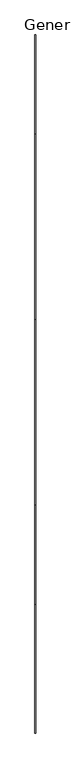
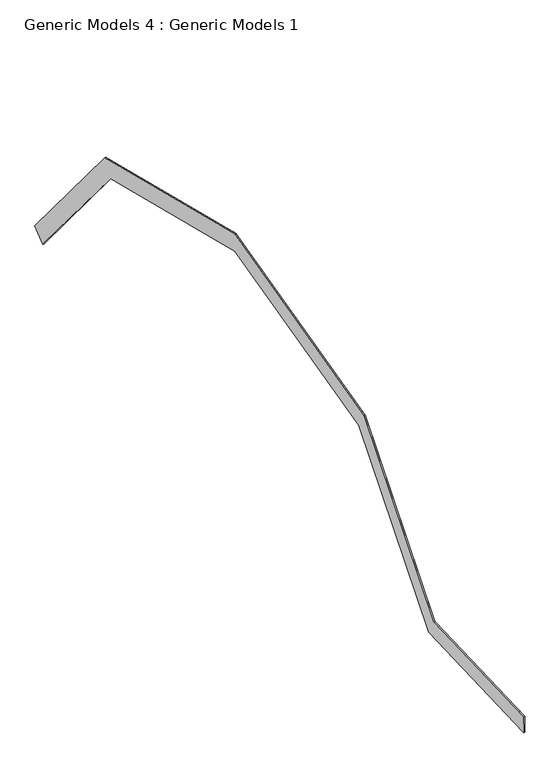
"""IFC4 building model written with IfcOpenShell, lengths in millimetres: proxy geometry, Generic Models 4 : Generic Models 1."""

from ifc_helpers import new_model, si_unit, frame, origin, place, context, project, spatial, polyline, outline, extrude, source, transform, mapped, element, save


def generic_models_4_generic_models_1_9f6939e7(model_context):
    return source(origin(), model_context, "Body", "SweptSolid", [
        extrude(outline(polyline([(11609.9309883, 2984.3405795), (10023.6412719, 4887.8882391), (7113.0570149, 5615.5343034), (4202.4384941, 4887.8796732), (2560.7151338, 2917.8116409), (331.5982071, 2831.1879261), (322.4759913, 3065.9329463), (2434.8673967, 3148.0206952), (4066.3626163, 5105.8149588), (7113.772024, 5867.6673107), (10161.1814316, 5105.8149588), (11797.360301, 3142.4003155), (11609.9309883, 2984.3405795)])), frame((29947.3870052, 0.0, 0.0), z_axis=(1.0, 0.0, 0.0), x_axis=(0.0, 1.0, 0.0)), (0.0, 0.0, 1.0), 13.5023771),
    ])


if __name__ == "__main__":
    model = new_model("IFC4")
    model_context = context("Model", 3, world=origin())
    ifc_project = project(units=[si_unit("LENGTHUNIT", "METRE", prefix="MILLI")], contexts=[model_context])
    site = spatial("IfcSite", under=ifc_project)
    building = spatial("IfcBuilding", under=site)
    placement = place(None, origin())
    generic_models_4_generic_models_1_shape = generic_models_4_generic_models_1_9f6939e7(model_context)
    element("IfcBuildingElementProxy", 1, Name="Generic Models 4 : Generic Models 1", ObjectType="Generic Models 4 : Generic Models 1", at=placement, inside=building, context=model_context, shape_type="MappedRepresentation", body=[
        mapped(generic_models_4_generic_models_1_shape, transform((0.0, 0.0, 0.0), x_axis=(1.0, 0.0, 0.0), y_axis=(0.0, 1.0, 0.0), z_axis=(0.0, 0.0, 1.0))),
    ])
    save(model, "model.ifc")
